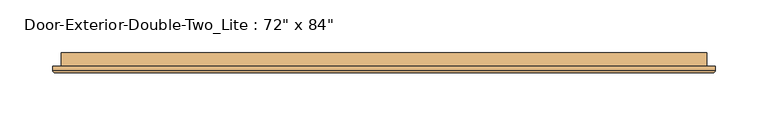
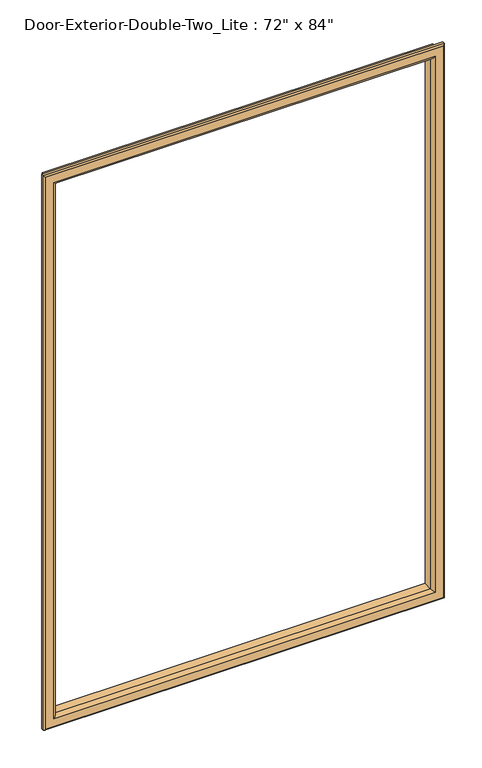
"""IFC4 building model written with IfcOpenShell, lengths in millimetres: door geometry."""

import ifcopenshell
import ifcopenshell.guid

model = None  # the IFC model being written
_history = None  # IfcOwnerHistory: only IFC2X3 demands one
_inside = {}  # id of a spatial element -> (the spatial element, [elements in it])
_under = {}  # id of a project, library or spatial element -> (it, [spatial elements below it])
_declared = {}  # id of a project -> (the project, [libraries it declares])
_typed = {}  # id of a type object -> (the type object, [elements of that type])
_made_of = {}  # id of a material, layer set ... -> (it, [elements and type objects made of it])


def new_model(schema):
    """Start an empty IFC model of exactly this schema.

    Asked for "IFC4X3", IfcOpenShell would pick the latest addendum, in which some entities
    have other attributes; the version numbers below select the first issue.
    IFC2X3 requires an IfcOwnerHistory on every rooted entity: one is made here for all.
    """
    global model, _history
    if schema == "IFC4X3":
        model = ifcopenshell.file(schema_version=(4, 3, 0, 0))
    else:
        model = ifcopenshell.file(schema=schema)
    _inside.clear()
    _under.clear()
    _declared.clear()
    _typed.clear()
    _made_of.clear()
    _history = None
    if model.schema == "IFC2X3":
        org = make("IfcOrganization", Name="unknown")
        user = make(
            "IfcPersonAndOrganization",
            ThePerson=make("IfcPerson", FamilyName="unknown"),
            TheOrganization=org,
        )
        app = make(
            "IfcApplication",
            ApplicationDeveloper=org,
            Version="unknown",
            ApplicationFullName="unknown",
            ApplicationIdentifier="unknown",
        )
        _history = make(
            "IfcOwnerHistory",
            OwningUser=user,
            OwningApplication=app,
            ChangeAction="ADDED",
            CreationDate=0,
        )
    return model


def make(cls, **values):
    """One entity of the class cls with the attributes given. An attribute that is None is left unset."""
    return model.create_entity(
        cls, **{name: value for name, value in values.items() if value is not None}
    )


def rooted(cls, **values):
    """An entity with a GlobalId (a new one), such as an element, a storey or a relation."""
    return make(cls, GlobalId=ifcopenshell.guid.new(), OwnerHistory=_history, **values)


def si_unit(unit_type, name, prefix=None):
    """IfcSIUnit, for example si_unit("LENGTHUNIT", "METRE", prefix="MILLI")."""
    return make("IfcSIUnit", UnitType=unit_type, Prefix=prefix, Name=name)


def assignment(units):
    """IfcUnitAssignment: the units of a project."""
    return None if units is None else make("IfcUnitAssignment", Units=units)


def point(xyz):
    """IfcCartesianPoint."""
    return None if xyz is None else make("IfcCartesianPoint", Coordinates=xyz)


def direction(xyz):
    """IfcDirection."""
    return None if xyz is None else make("IfcDirection", DirectionRatios=xyz)


def frame(location, z_axis=None, x_axis=None):
    """IfcAxis2Placement3D, a coordinate frame: its origin and axes. An axis left out is left unset."""
    return make(
        "IfcAxis2Placement3D",
        Location=point(location),
        Axis=direction(z_axis),
        RefDirection=direction(x_axis),
    )


def origin():
    """The frame at (0, 0, 0) with its axes left unset."""
    return frame((0.0, 0.0, 0.0))


def place(relative_to, where):
    """IfcLocalPlacement: puts the frame where relative to a parent placement (None: the world)."""
    return make(
        "IfcLocalPlacement", PlacementRelTo=relative_to, RelativePlacement=where
    )


def context(
    kind, dimensions, precision=None, world=None, true_north=None, identifier=None
):
    """IfcGeometricRepresentationContext, for example the 3D "Model" context."""
    return make(
        "IfcGeometricRepresentationContext",
        ContextIdentifier=identifier,
        ContextType=kind,
        CoordinateSpaceDimension=dimensions,
        Precision=precision,
        WorldCoordinateSystem=world,
        TrueNorth=true_north,
    )


def project(units=None, contexts=None):
    """IfcProject with its units and contexts."""
    return rooted(
        "IfcProject",
        Name="project",
        RepresentationContexts=contexts,
        UnitsInContext=assignment(units),
    )


def spatial(cls, under=None, at=None, **own):
    """A site, building, storey or space (cls), placed at a placement, below another one or the project."""
    s = rooted(cls, ObjectPlacement=at, **own)
    if under is not None:
        _under.setdefault(under.id(), (under, []))[1].append(s)
    return s


def ellipse_curve(where, semi_axis1, semi_axis2):
    """IfcEllipse in the frame where."""
    return make(
        "IfcEllipse", Position=where, SemiAxis1=semi_axis1, SemiAxis2=semi_axis2
    )


def shape(context_of_items, identifier, shape_type, items):
    """IfcShapeRepresentation: the items that make up one representation, for example the "Body"."""
    return make(
        "IfcShapeRepresentation",
        ContextOfItems=context_of_items,
        RepresentationIdentifier=identifier,
        RepresentationType=shape_type,
        Items=items,
    )


def source(mapping_origin, context_of_items, identifier, shape_type, items):
    """IfcRepresentationMap: a shape defined once, which mapped items show again and again."""
    return make(
        "IfcRepresentationMap",
        MappingOrigin=mapping_origin,
        MappedRepresentation=shape(context_of_items, identifier, shape_type, items),
    )


def transform(
    local_origin,
    x_axis=None,
    y_axis=None,
    z_axis=None,
    scale=None,
    scale2=None,
    scale3=None,
    uniform=True,
):
    """IfcCartesianTransformationOperator3D, or its non-uniform kind. x_axis, y_axis, z_axis: its Axis1, 2, 3."""
    if uniform:
        return make(
            "IfcCartesianTransformationOperator3D",
            Axis1=direction(x_axis),
            Axis2=direction(y_axis),
            LocalOrigin=point(local_origin),
            Scale=scale,
            Axis3=direction(z_axis),
        )
    return make(
        "IfcCartesianTransformationOperator3DnonUniform",
        Axis1=direction(x_axis),
        Axis2=direction(y_axis),
        LocalOrigin=point(local_origin),
        Scale=scale,
        Axis3=direction(z_axis),
        Scale2=scale2,
        Scale3=scale3,
    )


def mapped(mapping_source, mapping_target):
    """IfcMappedItem: shows the shape of a source again, moved by a transform."""
    return make(
        "IfcMappedItem", MappingSource=mapping_source, MappingTarget=mapping_target
    )


def made_of(thing, what):
    """Note that an element or type object is made of a material, layer set ...; save() writes the relation."""
    if what is not None:
        _made_of.setdefault(what.id(), (what, []))[1].append(thing)
    return thing


def element(
    cls,
    number,
    at=None,
    inside=None,
    cuts=None,
    type_object=None,
    material=None,
    context=None,
    identifier="Body",
    shape_type=None,
    held_by="IfcProductDefinitionShape",
    body=None,
    shapes=None,
    **own,
):
    """One element of the class cls, such as IfcWall. Its Tag is "e" and its number.

    at: its placement. inside: the storey or other place that contains it. cuts: it is an
    opening in that element (IfcRelVoidsElement). A single representation is given by context,
    identifier, shape_type and body (its items); several are given by shapes. held_by: the class
    of the entity that holds the representations. save() writes the other relations.
    """
    e = rooted(cls, Tag="e%d" % number, ObjectPlacement=at, **own)
    if body is not None:
        shapes = [shape(context, identifier, shape_type, body)]
    if shapes is not None:
        e.Representation = make(held_by, Representations=shapes)
    if inside is not None:
        _inside.setdefault(inside.id(), (inside, []))[1].append(e)
    if cuts is not None:
        rooted(
            "IfcRelVoidsElement", RelatingBuildingElement=cuts, RelatedOpeningElement=e
        )
    if type_object is not None:
        _typed.setdefault(type_object.id(), (type_object, []))[1].append(e)
    return made_of(e, material)


def aggregate(whole, parts):
    """IfcRelAggregates: a whole, such as a stair, and the parts it consists of."""
    return rooted("IfcRelAggregates", RelatingObject=whole, RelatedObjects=parts)


def save(model, path):
    """Write the relations noted so far, then the file.

    IfcRelAggregates (storeys below a building ...), IfcRelContainedInSpatialStructure (elements
    in a storey), IfcRelDefinesByType, IfcRelAssociatesMaterial and IfcRelDeclares: one each for
    every whole, place, type object, material and project.
    """
    for whole, parts in _under.values():
        aggregate(whole, parts)
    for where, things in _inside.values():
        rooted(
            "IfcRelContainedInSpatialStructure",
            RelatedElements=things,
            RelatingStructure=where,
        )
    for kind, things in _typed.values():
        rooted("IfcRelDefinesByType", RelatedObjects=things, RelatingType=kind)
    for what, things in _made_of.values():
        rooted("IfcRelAssociatesMaterial", RelatedObjects=things, RelatingMaterial=what)
    for by, libraries in _declared.values():
        rooted("IfcRelDeclares", RelatingContext=by, RelatedDefinitions=libraries)
    model.write(path)


def plane_surface(at):
    """IfcPlane: the flat surface through the origin of the frame at, square to its z axis."""
    return make("IfcPlane", Position=at)


def cylinder_surface(at, radius):
    """IfcCylindricalSurface: all points at the distance radius from the z axis of the frame at."""
    return make("IfcCylindricalSurface", Position=at, Radius=radius)


def advanced_brep(points, edges, surfaces, faces):
    """IfcAdvancedBrep: a solid bounded by faces that lie on surfaces and meet in shared edges.

    An edge is (start, end): straight between two places in points (the first is 0);
    or (start, end, curve); or (start, end, curve, False) where it runs against its curve.
    A face is (place in surfaces, loops), or (place, loops, False) where it looks against
    its surface's normal. A loop lists edges by number (the first is 1), with a minus sign
    where the edge is run from its end to its start. The first loop is the outer one.
    """
    corners = [point(p) for p in points]
    vertices = [make("IfcVertexPoint", VertexGeometry=c) for c in corners]
    made = []
    for start, end, *more in edges:
        made.append(
            make(
                "IfcEdgeCurve",
                EdgeStart=vertices[start],
                EdgeEnd=vertices[end],
                EdgeGeometry=more[0] if more else make("IfcPolyline", Points=[corners[start], corners[end]]),
                SameSense=more[1] if len(more) > 1 else True,
            )
        )
    hull = []
    for where, loops, *sense in faces:
        bounds = []
        for j, loop in enumerate(loops):
            ring = [make("IfcOrientedEdge", EdgeElement=made[abs(k) - 1], Orientation=k > 0) for k in loop]
            bounds.append(
                make(
                    "IfcFaceOuterBound" if j == 0 else "IfcFaceBound",
                    Bound=make("IfcEdgeLoop", EdgeList=ring),
                    Orientation=True,
                )
            )
        hull.append(make("IfcAdvancedFace", Bounds=bounds, FaceSurface=surfaces[where], SameSense=sense[0] if sense else True))
    return make("IfcAdvancedBrep", Outer=make("IfcClosedShell", CfsFaces=hull))


def door_d7bfd8b5(model_context):
    return source(origin(), model_context, "Body", "AdvancedBrep", [
        advanced_brep(
        [(-762.0, 52.3875, 1117.6), (-762.0, 39.6875, 1117.6), (-762.0, 39.6875, 2016.125), (-762.0, 52.3875, 2016.125), (-750.0, 38.6875, 1129.6), (-750.0, 52.3875, 1129.6), (-750.0, 52.3875, 2004.125), (-750.0, 38.6875, 2004.125), (-755.0, 33.6875, 1124.6), (-755.0, 33.6875, 2009.125), (-770.0, 35.6875, 1109.6), (-768.0, 33.6875, 1111.6), (-768.0, 33.6875, 2022.125), (-770.0, 35.6875, 2024.125), (-770.0, 39.6875, 1109.6), (-770.0, 39.6875, 2024.125), (-152.4, 39.6875, 2016.125), (-152.4, 52.3875, 2016.125), (-164.4, 52.3875, 2004.125), (-164.4, 38.6875, 2004.125), (-159.4, 33.6875, 2009.125), (-146.4, 33.6875, 2022.125), (-144.4, 35.6875, 2024.125), (-144.4, 39.6875, 2024.125), (-152.4, 39.6875, 1117.6), (-152.4, 52.3875, 1117.6), (-164.4, 52.3875, 1129.6), (-164.4, 38.6875, 1129.6), (-159.4, 33.6875, 1124.6), (-146.4, 33.6875, 1111.6), (-144.4, 35.6875, 1109.6), (-144.4, 39.6875, 1109.6)],
        [
            (0, 1),
            (1, 2),
            (2, 3),
            (3, 0),
            (4, 5),
            (5, 6),
            (6, 7),
            (7, 4),
            (8, 4, ellipse_curve(frame((-755.0, 38.6875, 1124.6), z_axis=(-0.7071067811865475, 0.0, 0.7071067811865475), x_axis=(-0.7071067811865474, 0.0, -0.7071067811865476)), 7.0710678, 5.0)),
            (7, 9, ellipse_curve(frame((-755.0, 38.6875, 2009.125), z_axis=(-0.7071067811865475, 0.0, -0.7071067811865475), x_axis=(0.7071067811865474, 0.0, -0.7071067811865476)), 7.0710678, 5.0)),
            (9, 8),
            (10, 11, ellipse_curve(frame((-768.0, 35.6875, 1111.6), z_axis=(-0.7071067811865475, 0.0, 0.7071067811865475), x_axis=(-0.7071067811865474, 0.0, -0.7071067811865476)), 2.8284271, 2.0)),
            (11, 12),
            (12, 13, ellipse_curve(frame((-768.0, 35.6875, 2022.125), z_axis=(-0.7071067811865475, 0.0, -0.7071067811865475), x_axis=(0.7071067811865474, 0.0, -0.7071067811865476)), 2.8284271, 2.0)),
            (13, 10),
            (14, 10),
            (13, 15),
            (15, 14),
            (2, 16),
            (16, 17),
            (17, 3),
            (6, 18),
            (18, 19),
            (19, 7),
            (19, 20, ellipse_curve(frame((-159.4, 38.6875, 2009.125), z_axis=(-0.7071067811865475, 0.0, 0.7071067811865475), x_axis=(-0.7071067811865476, 0.0, -0.7071067811865474)), 7.0710678, 5.0)),
            (20, 9),
            (12, 21),
            (21, 22, ellipse_curve(frame((-146.4, 35.6875, 2022.125), z_axis=(-0.7071067811865475, 0.0, 0.7071067811865475), x_axis=(-0.7071067811865476, 0.0, -0.7071067811865474)), 2.8284271, 2.0)),
            (22, 13),
            (22, 23),
            (23, 15),
            (16, 24),
            (24, 25),
            (25, 17),
            (18, 26),
            (26, 27),
            (27, 19),
            (27, 28, ellipse_curve(frame((-159.4, 38.6875, 1124.6), z_axis=(0.7071067811865475, 0.0, 0.7071067811865475), x_axis=(-0.7071067811865474, 0.0, 0.7071067811865476)), 7.0710678, 5.0)),
            (28, 20),
            (21, 29),
            (29, 30, ellipse_curve(frame((-146.4, 35.6875, 1111.6), z_axis=(0.7071067811865475, 0.0, 0.7071067811865475), x_axis=(-0.7071067811865474, 0.0, 0.7071067811865476)), 2.8284271, 2.0)),
            (30, 22),
            (30, 31),
            (31, 23),
            (31, 14),
            (1, 24),
            (0, 25),
            (5, 26),
            (4, 27),
            (8, 28),
            (11, 29),
            (10, 30),
        ],
        [
            plane_surface(frame((-762.0, 39.6875, 1117.6), z_axis=(-1.0, 0.0, 0.0), x_axis=(0.0, 0.0, 1.0))),
            plane_surface(frame((-750.0, 52.3875, 1129.6), z_axis=(1.0, 0.0, 0.0), x_axis=(0.0, 0.0, 1.0))),
            cylinder_surface(frame((-755.0, 38.6875, 1117.6), z_axis=(0.0, 0.0, -1.0), x_axis=(-1.0, 0.0, 0.0)), 5.0),
            cylinder_surface(frame((-768.0, 35.6875, 1117.6), z_axis=(0.0, 0.0, -1.0), x_axis=(-1.0, 0.0, 0.0)), 2.0),
            plane_surface(frame((-770.0, 35.6875, 1109.6), z_axis=(-1.0, 0.0, 0.0), x_axis=(0.0, 0.0, 1.0))),
            plane_surface(frame((-762.0, 39.6875, 2016.125), z_axis=(0.0, 0.0, 1.0), x_axis=(1.0, 0.0, 0.0))),
            plane_surface(frame((-750.0, 52.3875, 2004.125), z_axis=(0.0, 0.0, -1.0), x_axis=(1.0, 0.0, 0.0))),
            cylinder_surface(frame((-762.0, 38.6875, 2009.125), z_axis=(-1.0, 0.0, 0.0), x_axis=(0.0, 0.0, 1.0)), 5.0),
            cylinder_surface(frame((-762.0, 35.6875, 2022.125), z_axis=(-1.0, 0.0, 0.0), x_axis=(0.0, 0.0, 1.0)), 2.0),
            plane_surface(frame((-770.0, 35.6875, 2024.125), z_axis=(0.0, 0.0, 1.0), x_axis=(1.0, 0.0, 0.0))),
            plane_surface(frame((-152.4, 39.6875, 2016.125), z_axis=(1.0, 0.0, 0.0), x_axis=(0.0, 0.0, -1.0))),
            plane_surface(frame((-164.4, 52.3875, 2004.125), z_axis=(-1.0, 0.0, 0.0), x_axis=(0.0, 0.0, -1.0))),
            cylinder_surface(frame((-159.4, 38.6875, 2016.125), z_axis=(0.0, 0.0, 1.0), x_axis=(1.0, 0.0, 0.0)), 5.0),
            cylinder_surface(frame((-146.4, 35.6875, 2016.125), z_axis=(0.0, 0.0, 1.0), x_axis=(1.0, 0.0, 0.0)), 2.0),
            plane_surface(frame((-144.4, 35.6875, 2024.125), z_axis=(1.0, 0.0, 0.0), x_axis=(0.0, 0.0, -1.0))),
            plane_surface(frame((-144.4, 39.6875, 1109.6), z_axis=(0.0, 1.0, 0.0), x_axis=(-1.0, 0.0, 0.0))),
            plane_surface(frame((-152.4, 39.6875, 1117.6), z_axis=(0.0, 0.0, -1.0), x_axis=(-1.0, 0.0, 0.0))),
            plane_surface(frame((-152.4, 52.3875, 1117.6), z_axis=(0.0, 1.0, 0.0), x_axis=(-1.0, 0.0, 0.0))),
            plane_surface(frame((-164.4, 52.3875, 1129.6), z_axis=(0.0, 0.0, 1.0), x_axis=(-1.0, 0.0, 0.0))),
            cylinder_surface(frame((-152.4, 38.6875, 1124.6), z_axis=(1.0, 0.0, 0.0), x_axis=(0.0, 0.0, -1.0)), 5.0),
            plane_surface(frame((-159.4, 33.6875, 1124.6), z_axis=(0.0, -1.0, 0.0), x_axis=(-1.0, 0.0, 0.0))),
            cylinder_surface(frame((-152.4, 35.6875, 1111.6), z_axis=(1.0, 0.0, 0.0), x_axis=(0.0, 0.0, -1.0)), 2.0),
            plane_surface(frame((-144.4, 35.6875, 1109.6), z_axis=(0.0, 0.0, -1.0), x_axis=(-1.0, 0.0, 0.0))),
        ],
        [
            (0, [[1, 2, 3, 4]]),
            (1, [[5, 6, 7, 8]]),
            (2, [[9, -8, 10, 11]]),
            (3, [[12, 13, 14, 15]]),
            (4, [[16, -15, 17, 18]]),
            (5, [[-3, 19, 20, 21]]),
            (6, [[-7, 22, 23, 24]]),
            (7, [[-10, -24, 25, 26]]),
            (8, [[-14, 27, 28, 29]]),
            (9, [[-17, -29, 30, 31]]),
            (10, [[-20, 32, 33, 34]]),
            (11, [[-23, 35, 36, 37]]),
            (12, [[-25, -37, 38, 39]]),
            (13, [[-28, 40, 41, 42]]),
            (14, [[-30, -42, 43, 44]]),
            (15, [[-31, -44, 45, -18], [46, -32, -19, -2]]),
            (16, [[-33, -46, -1, 47]]),
            (17, [[-21, -34, -47, -4], [48, -35, -22, -6]]),
            (18, [[-36, -48, -5, 49]]),
            (19, [[-38, -49, -9, 50]]),
            (20, [[51, -40, -27, -13], [-26, -39, -50, -11]]),
            (21, [[-41, -51, -12, 52]]),
            (22, [[-43, -52, -16, -45]]),
        ],
    ),
    ])


if __name__ == "__main__":
    model = new_model("IFC4")
    model_context = context("Model", 3, world=origin())
    ifc_project = project(units=[si_unit("LENGTHUNIT", "METRE", prefix="MILLI")], contexts=[model_context])
    site = spatial("IfcSite", under=ifc_project)
    building = spatial("IfcBuilding", under=site)
    placement = place(None, origin())
    door_shape = door_d7bfd8b5(model_context)
    element("IfcDoor", 1, ObjectType="Door-Exterior-Double-Two_Lite : 72\" x 84\"", at=placement, inside=building, context=model_context, shape_type="MappedRepresentation", body=[
        mapped(door_shape, transform((0.0, 0.0, 0.0), x_axis=(1.0, 0.0, 0.0), y_axis=(0.0, 1.0, 0.0), z_axis=(0.0, 0.0, 1.0))),
    ])
    save(model, "model.ifc")

# Revit data of these elements
# Type "Door-Exterior-Double-Two_Lite : 72\" x 84\""
#   Type Mark = "20"
#   Assembly Code = "B2030100"
#   Analytic Construction = "Metal frame, double glass door"
#   Top Rail = 0' - 4 5/8"
#   Threshold Length [instance default] = 6' - 4"
#   Threshold Offset [instance default] = 0' - 0 1/2"
#   Thickness = 0' - 1 3/4"
#   Thermal Resistance (R) = 1.3794 (h·ft²·°F)/BTU
#   Swing Angle [instance default] = 90.00°
#   Strike Height = 3' - 4"
#   Stiles = 0' - 6"
#   SinglePanelWidth = 3' - 0"
#   Rough Width [instance default] = 6' - 4"
#   Rough Height [instance default] = 7' - 4"
#   MFOpeningHeight [instance default] = 0' - 4"
#   MFOpeningWidth [instance default] = 0' - 4"
#   Lock Rail = 0' - 8"
#   Inset Calculate [instance default] = 0' - 4"
#   Masonry Inset [instance default] = 0' - 1"
#   Height = 7' - 0"
#   Width = 6' - 0"
#   Heat Transfer Coefficient (U) = 0.7250 BTU/(h·ft²·°F)
#   Glass Thickness = 0' - 0 3/4"
#   Masonry Frame Depth = 0' - 5 3/4"
#   Bottom Rail = 0' - 10"
#   Threshold [instance default] = yes
#   Masonry Frame [instance default] = yes
#   Function = 1
#   Dry Wall Frame [instance default] = no
#   Threshold Material = none
#   Panic Bar Material = Metal - Stainless Steel
#   Panel Material = Metal - Painted - Grey
#   Glass Stop Material = Metal - Painted - Grey
#   Frame Material = Metal - Painted - Grey
#   Exterior Pull Material = Metal - Stainless Steel
#   Visual Light Transmittance = 0
#   Solar Heat Gain Coefficient = 0
#   Wall Closure = (empty or 0)
# Element 1 (IfcDoor, "Door-Exterior-Double-Two_Lite : 72\" x 84\"")
#   Threshold Length = 6' - 0"
#   Rough Width = 6' - 2 1/2"
#   Rough Height = 7' - 1 1/4"
#   MFOpeningHeight = 0' - 1 1/4"
#   MFOpeningWidth = 0' - 2 1/2"
#   Inset Calculate = 0' - 3"
#   Masonry Frame = no
#   Dry Wall Frame = yes
#   Materials on its faces: "Metal - Painted - Grey", "Metal - Stainless Steel", "Glass"
# Materials
#   "Metal - Stainless Steel": class "Metal", colour RGB 247 247 247, transparency 0
#   "Metal - Painted - Grey": class "Paint", colour RGB 104 104 104, transparency 0, Cost = 0
#   "Glass": class "Glass", colour RGB 0 128 192, transparency 0.75, Description = "Soda Lime Glass", Cost = 0
